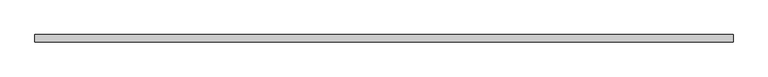
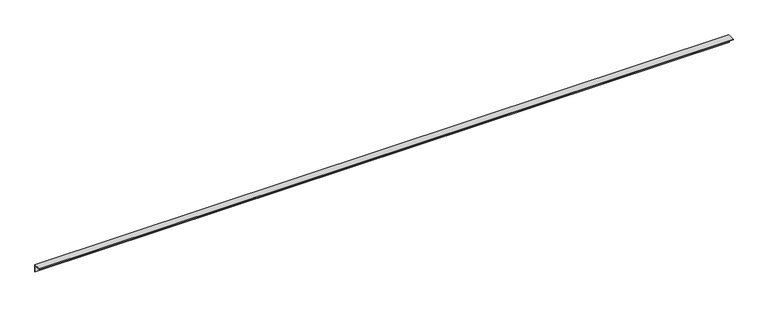
"""IFC4 building model written with IfcOpenShell, lengths in millimetres: proxy geometry, Generic Models 7:Generic Models 1:337419:Generic Models 1:337419 : Generic Models 7:Generic Models 1:337419:5 : Generic Models 7:Generic Models 1:337419:Generic Models 1:337419 : Generic Models 7:Generic Models 1:337419:301336."""

from ifc_helpers import new_model, si_unit, frame, origin, place, context, project, spatial, polyline, outline, extrude, source, transform, mapped, element, save


def generic_models_4e93bdbc(model_context):
    return source(origin(), model_context, "Body", "SweptSolid", [
        extrude(outline(polyline([(-568189.8163841, 4903.0824276), (-568189.8163841, 4852.2824276), (-568194.5788841, 4852.2824276), (-568194.5788841, 4898.3199276), (-568240.6163841, 4898.3199276), (-568240.6163841, 4903.0824276), (-568189.8163841, 4903.0824276)])), frame((591306.0367242, 0.0, 0.0), z_axis=(1.0, 0.0, 0.0), x_axis=(0.0, 1.0, 0.0)), (0.0, 0.0, 1.0), 4876.8),
    ])


if __name__ == "__main__":
    model = new_model("IFC4")
    model_context = context("Model", 3, world=origin())
    ifc_project = project(units=[si_unit("LENGTHUNIT", "METRE", prefix="MILLI")], contexts=[model_context])
    site = spatial("IfcSite", under=ifc_project)
    building = spatial("IfcBuilding", under=site)
    placement = place(None, origin())
    generic_models_shape = generic_models_4e93bdbc(model_context)
    element("IfcBuildingElementProxy", 1, Name="Generic Models 7:Generic Models 1:337419:Generic Models 1:337419 : Generic Models 7:Generic Models 1:337419:5 : Generic Models 7:Generic Models 1:337419:Generic Models 1:337419 : Generic Models 7:Generic Models 1:337419:301336", ObjectType="Generic Models 7:Generic Models 1:337419:Generic Models 1:337419 : Generic Models 7:Generic Models 1:337419:5 : Generic Models 7:Generic Models 1:337419:Generic Models 1:337419 : Generic Models 7:Generic Models 1:337419:301336", at=placement, inside=building, context=model_context, shape_type="MappedRepresentation", body=[
        mapped(generic_models_shape, transform((0.0, 0.0, 0.0), x_axis=(1.0, 0.0, 0.0), y_axis=(0.0, 1.0, 0.0), z_axis=(0.0, 0.0, 1.0))),
    ])
    save(model, "model.ifc")

# Revit data of these elements
# Type "Generic Models 7:Generic Models 1:337419:Generic Models 1:337419 : Generic Models 7:Generic Models 1:337419:5 : Generic Models 7:Generic Models 1:337419:Generic Models 1:337419 : Generic Models 7:Generic Models 1:337419:301336"
#   NameOverride = "Generic Models 7:Generic Models 1:337419:Generic Models 1:337419 : Generic Models 7:Generic Models 1:337419:301336"
#   ObjectTypeOverride = "Generic Models 1:337419 : Generic Models 7:Generic Models 1:337419"
#   Reference = "Generic Models 1"
#   Tag = "301336"
# Element 1 (IfcBuildingElementProxy, "Generic Models 7:Generic Models 1:337419:Generic Models 1:337419 : Generic Models 7:Generic Models 1:337419:5 : Generic Models 7:Generic Models 1:337419:Generic Models 1:337419 : Generic Models 7:Generic Models 1:337419:301336")
#   Materials on its faces: "GALVANIZED STEEL ANGLE (L2x2x1/4) WITH #12 GRADE 5 SCREWS @ 24\" O.C."
# Materials
#   "GALVANIZED STEEL ANGLE (L2x2x1/4) WITH #12 GRADE 5 SCREWS @ 24\" O.C.": class "Unassigned", colour RGB 210 209 208, transparency 0, Keynote = "M05121300.02", Cost = 0
